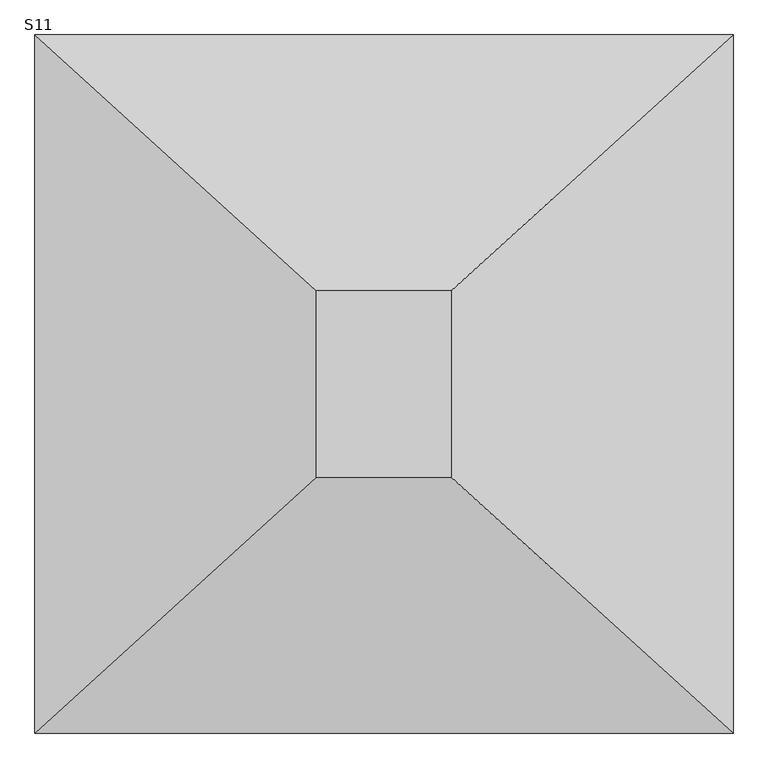
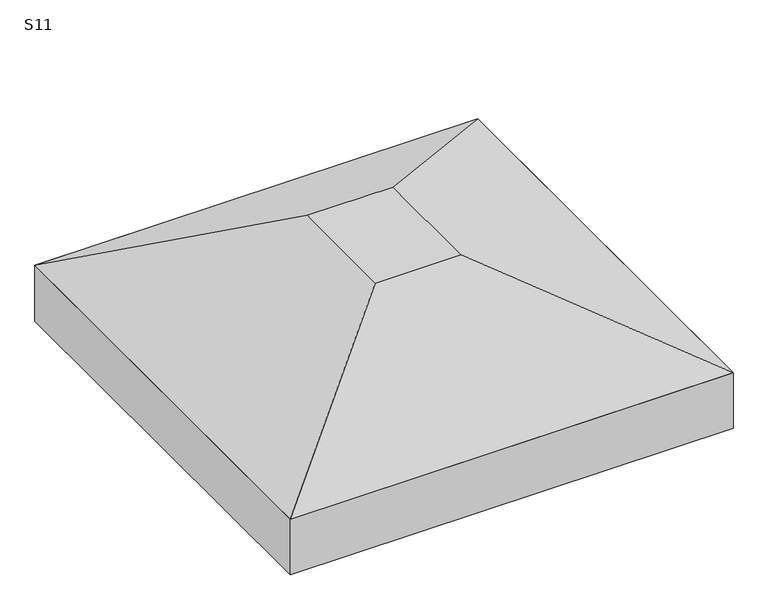
"""IFC4 building model written with IfcOpenShell, lengths in millimetres: fastener geometry, TQS - Sapata : S11."""

import ifcopenshell
import ifcopenshell.guid

model = None  # the IFC model being written
_history = None  # IfcOwnerHistory: only IFC2X3 demands one
_inside = {}  # id of a spatial element -> (the spatial element, [elements in it])
_under = {}  # id of a project, library or spatial element -> (it, [spatial elements below it])
_declared = {}  # id of a project -> (the project, [libraries it declares])
_typed = {}  # id of a type object -> (the type object, [elements of that type])
_made_of = {}  # id of a material, layer set ... -> (it, [elements and type objects made of it])


def new_model(schema):
    """Start an empty IFC model of exactly this schema.

    Asked for "IFC4X3", IfcOpenShell would pick the latest addendum, in which some entities
    have other attributes; the version numbers below select the first issue.
    IFC2X3 requires an IfcOwnerHistory on every rooted entity: one is made here for all.
    """
    global model, _history
    if schema == "IFC4X3":
        model = ifcopenshell.file(schema_version=(4, 3, 0, 0))
    else:
        model = ifcopenshell.file(schema=schema)
    _inside.clear()
    _under.clear()
    _declared.clear()
    _typed.clear()
    _made_of.clear()
    _history = None
    if model.schema == "IFC2X3":
        org = make("IfcOrganization", Name="unknown")
        user = make(
            "IfcPersonAndOrganization",
            ThePerson=make("IfcPerson", FamilyName="unknown"),
            TheOrganization=org,
        )
        app = make(
            "IfcApplication",
            ApplicationDeveloper=org,
            Version="unknown",
            ApplicationFullName="unknown",
            ApplicationIdentifier="unknown",
        )
        _history = make(
            "IfcOwnerHistory",
            OwningUser=user,
            OwningApplication=app,
            ChangeAction="ADDED",
            CreationDate=0,
        )
    return model


def make(cls, **values):
    """One entity of the class cls with the attributes given. An attribute that is None is left unset."""
    return model.create_entity(
        cls, **{name: value for name, value in values.items() if value is not None}
    )


def rooted(cls, **values):
    """An entity with a GlobalId (a new one), such as an element, a storey or a relation."""
    return make(cls, GlobalId=ifcopenshell.guid.new(), OwnerHistory=_history, **values)


def si_unit(unit_type, name, prefix=None):
    """IfcSIUnit, for example si_unit("LENGTHUNIT", "METRE", prefix="MILLI")."""
    return make("IfcSIUnit", UnitType=unit_type, Prefix=prefix, Name=name)


def assignment(units):
    """IfcUnitAssignment: the units of a project."""
    return None if units is None else make("IfcUnitAssignment", Units=units)


def point(xyz):
    """IfcCartesianPoint."""
    return None if xyz is None else make("IfcCartesianPoint", Coordinates=xyz)


def direction(xyz):
    """IfcDirection."""
    return None if xyz is None else make("IfcDirection", DirectionRatios=xyz)


def frame(location, z_axis=None, x_axis=None):
    """IfcAxis2Placement3D, a coordinate frame: its origin and axes. An axis left out is left unset."""
    return make(
        "IfcAxis2Placement3D",
        Location=point(location),
        Axis=direction(z_axis),
        RefDirection=direction(x_axis),
    )


def origin():
    """The frame at (0, 0, 0) with its axes left unset."""
    return frame((0.0, 0.0, 0.0))


def place(relative_to, where):
    """IfcLocalPlacement: puts the frame where relative to a parent placement (None: the world)."""
    return make(
        "IfcLocalPlacement", PlacementRelTo=relative_to, RelativePlacement=where
    )


def context(
    kind, dimensions, precision=None, world=None, true_north=None, identifier=None
):
    """IfcGeometricRepresentationContext, for example the 3D "Model" context."""
    return make(
        "IfcGeometricRepresentationContext",
        ContextIdentifier=identifier,
        ContextType=kind,
        CoordinateSpaceDimension=dimensions,
        Precision=precision,
        WorldCoordinateSystem=world,
        TrueNorth=true_north,
    )


def project(units=None, contexts=None):
    """IfcProject with its units and contexts."""
    return rooted(
        "IfcProject",
        Name="project",
        RepresentationContexts=contexts,
        UnitsInContext=assignment(units),
    )


def spatial(cls, under=None, at=None, **own):
    """A site, building, storey or space (cls), placed at a placement, below another one or the project."""
    s = rooted(cls, ObjectPlacement=at, **own)
    if under is not None:
        _under.setdefault(under.id(), (under, []))[1].append(s)
    return s


def polyline(points):
    """IfcPolyline through the points."""
    return make("IfcPolyline", Points=[point(p) for p in points])


def outline(outer, holes=None, kind="AREA"):
    """IfcArbitraryClosedProfileDef: a profile drawn as a closed curve; with holes, ...WithVoids."""
    if holes is None:
        return make("IfcArbitraryClosedProfileDef", ProfileType=kind, OuterCurve=outer)
    return make(
        "IfcArbitraryProfileDefWithVoids",
        ProfileType=kind,
        OuterCurve=outer,
        InnerCurves=holes,
    )


def extrude(swept, where, along, depth):
    """IfcExtrudedAreaSolid: the profile swept, set in the frame where, extruded along a direction by depth."""
    return make(
        "IfcExtrudedAreaSolid",
        SweptArea=swept,
        Position=where,
        ExtrudedDirection=direction(along),
        Depth=depth,
    )


def faces_of(points, faces, orient=None, outer=None):
    """IfcFace entities. A face is a list of loops; a loop is a list of indices into points, from 0.

    orient and outer hold one flag for each loop. By default every Orientation is true, the
    first loop of a face is its IfcFaceOuterBound and the others are IfcFaceBound.
    """
    made = []
    for i, loops in enumerate(faces):
        bounds = []
        for j, loop in enumerate(loops):
            is_outer = j == 0 if outer is None else outer[i][j]
            bounds.append(
                make(
                    "IfcFaceOuterBound" if is_outer else "IfcFaceBound",
                    Bound=make("IfcPolyLoop", Polygon=[points[k] for k in loop]),
                    Orientation=True if orient is None else orient[i][j],
                )
            )
        made.append(make("IfcFace", Bounds=bounds))
    return made


def faceted_brep(points, faces, orient=None, outer=None, voids=None):
    """IfcFacetedBrep: a solid bounded by flat faces; with voids (closed shells), ...WithVoids."""
    shared = [point(p) for p in points]
    hull = make("IfcClosedShell", CfsFaces=faces_of(shared, faces, orient, outer))
    if voids is None:
        return make("IfcFacetedBrep", Outer=hull)
    return make(
        "IfcFacetedBrepWithVoids",
        Outer=hull,
        Voids=[
            make(cls, CfsFaces=faces_of(shared, fs, o, b)) for cls, fs, o, b in voids
        ],
    )


def shape(context_of_items, identifier, shape_type, items):
    """IfcShapeRepresentation: the items that make up one representation, for example the "Body"."""
    return make(
        "IfcShapeRepresentation",
        ContextOfItems=context_of_items,
        RepresentationIdentifier=identifier,
        RepresentationType=shape_type,
        Items=items,
    )


def source(mapping_origin, context_of_items, identifier, shape_type, items):
    """IfcRepresentationMap: a shape defined once, which mapped items show again and again."""
    return make(
        "IfcRepresentationMap",
        MappingOrigin=mapping_origin,
        MappedRepresentation=shape(context_of_items, identifier, shape_type, items),
    )


def transform(
    local_origin,
    x_axis=None,
    y_axis=None,
    z_axis=None,
    scale=None,
    scale2=None,
    scale3=None,
    uniform=True,
):
    """IfcCartesianTransformationOperator3D, or its non-uniform kind. x_axis, y_axis, z_axis: its Axis1, 2, 3."""
    if uniform:
        return make(
            "IfcCartesianTransformationOperator3D",
            Axis1=direction(x_axis),
            Axis2=direction(y_axis),
            LocalOrigin=point(local_origin),
            Scale=scale,
            Axis3=direction(z_axis),
        )
    return make(
        "IfcCartesianTransformationOperator3DnonUniform",
        Axis1=direction(x_axis),
        Axis2=direction(y_axis),
        LocalOrigin=point(local_origin),
        Scale=scale,
        Axis3=direction(z_axis),
        Scale2=scale2,
        Scale3=scale3,
    )


def mapped(mapping_source, mapping_target):
    """IfcMappedItem: shows the shape of a source again, moved by a transform."""
    return make(
        "IfcMappedItem", MappingSource=mapping_source, MappingTarget=mapping_target
    )


def made_of(thing, what):
    """Note that an element or type object is made of a material, layer set ...; save() writes the relation."""
    if what is not None:
        _made_of.setdefault(what.id(), (what, []))[1].append(thing)
    return thing


def element(
    cls,
    number,
    at=None,
    inside=None,
    cuts=None,
    type_object=None,
    material=None,
    context=None,
    identifier="Body",
    shape_type=None,
    held_by="IfcProductDefinitionShape",
    body=None,
    shapes=None,
    **own,
):
    """One element of the class cls, such as IfcWall. Its Tag is "e" and its number.

    at: its placement. inside: the storey or other place that contains it. cuts: it is an
    opening in that element (IfcRelVoidsElement). A single representation is given by context,
    identifier, shape_type and body (its items); several are given by shapes. held_by: the class
    of the entity that holds the representations. save() writes the other relations.
    """
    e = rooted(cls, Tag="e%d" % number, ObjectPlacement=at, **own)
    if body is not None:
        shapes = [shape(context, identifier, shape_type, body)]
    if shapes is not None:
        e.Representation = make(held_by, Representations=shapes)
    if inside is not None:
        _inside.setdefault(inside.id(), (inside, []))[1].append(e)
    if cuts is not None:
        rooted(
            "IfcRelVoidsElement", RelatingBuildingElement=cuts, RelatedOpeningElement=e
        )
    if type_object is not None:
        _typed.setdefault(type_object.id(), (type_object, []))[1].append(e)
    return made_of(e, material)


def aggregate(whole, parts):
    """IfcRelAggregates: a whole, such as a stair, and the parts it consists of."""
    return rooted("IfcRelAggregates", RelatingObject=whole, RelatedObjects=parts)


def save(model, path):
    """Write the relations noted so far, then the file.

    IfcRelAggregates (storeys below a building ...), IfcRelContainedInSpatialStructure (elements
    in a storey), IfcRelDefinesByType, IfcRelAssociatesMaterial and IfcRelDeclares: one each for
    every whole, place, type object, material and project.
    """
    for whole, parts in _under.values():
        aggregate(whole, parts)
    for where, things in _inside.values():
        rooted(
            "IfcRelContainedInSpatialStructure",
            RelatedElements=things,
            RelatingStructure=where,
        )
    for kind, things in _typed.values():
        rooted("IfcRelDefinesByType", RelatedObjects=things, RelatingType=kind)
    for what, things in _made_of.values():
        rooted("IfcRelAssociatesMaterial", RelatedObjects=things, RelatingMaterial=what)
    for by, libraries in _declared.values():
        rooted("IfcRelDeclares", RelatingContext=by, RelatedDefinitions=libraries)
    model.write(path)


def s11_36e66e76(model_context):
    return source(origin(), model_context, "Body", "SolidModel", [
        faceted_brep([(-55.0, 0.0, 0.0), (-345.0, 0.0, 0.0), (-345.0, -400.0, 0.0), (-55.0, -400.0, 0.0), (550.0, 550.0, -300.0), (550.0, -950.0, -300.0), (-950.0, -950.0, -300.0), (-950.0, 550.0, -300.0)], [[[0, 1, 2, 3]], [[4, 5, 6, 7]], [[4, 7, 1, 0]], [[7, 6, 2, 1]], [[6, 5, 3, 2]], [[5, 4, 0, 3]]]),
        extrude(outline(polyline([(550.0, 550.0), (550.0, -950.0), (-950.0, -950.0), (-950.0, 550.0), (550.0, 550.0)])), frame((0.0, 0.0, -500.0), z_axis=(0.0, 0.0, 1.0), x_axis=(1.0, 0.0, 0.0)), (0.0, 0.0, 1.0), 200.0),
    ])


if __name__ == "__main__":
    model = new_model("IFC4")
    model_context = context("Model", 3, world=origin())
    ifc_project = project(units=[si_unit("LENGTHUNIT", "METRE", prefix="MILLI")], contexts=[model_context])
    site = spatial("IfcSite", under=ifc_project)
    building = spatial("IfcBuilding", under=site)
    placement = place(None, origin())
    s11_shape = s11_36e66e76(model_context)
    element("IfcFastener", 1, ObjectType="TQS - Sapata : S11", at=placement, inside=building, context=model_context, shape_type="MappedRepresentation", body=[
        mapped(s11_shape, transform((0.0, 0.0, 0.0), x_axis=(1.0, 0.0, 0.0), y_axis=(0.0, 1.0, 0.0), z_axis=(0.0, 0.0, 1.0))),
    ])
    save(model, "model.ifc")

# Revit data of these elements
# Type "TQS - Sapata : S11"
#   TY = 0.40 m
#   TX = 0.29 m
#   HS = 0.50 m
#   H0 = 0.20 m
#   EXCYABS = 0.75 m
#   EXCY = 0.00 m
#   EXCXABS = 0.75 m
#   EXCX = 0.00 m
#   DIMY = 1.50 m
#   DIMX = 1.50 m
#   Material estrutural = Concreto - Concreto concretado no local
#   Width = 0
#   Length = 0
# Element 1 (IfcFastener, "TQS - Sapata : S11")
#   Materials on its faces: "Concreto - Concreto concretado no local"
# Materials
#   "Concreto - Concreto concretado no local": class "Concreto", colour RGB 192 192 192, transparency 0
